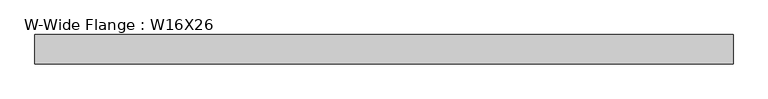
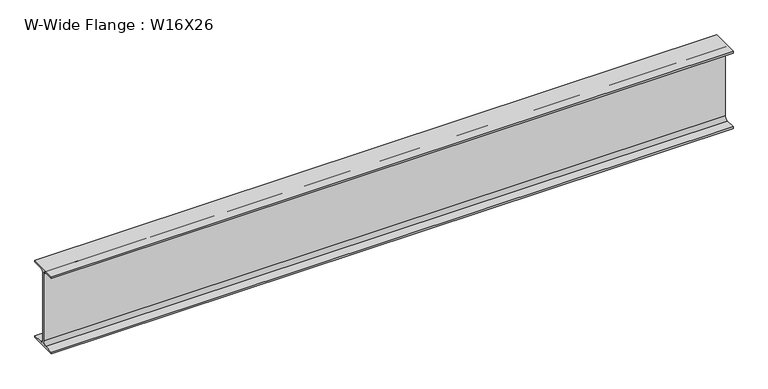
"""IFC4 building model written with IfcOpenShell, lengths in millimetres: beam geometry, W-Wide Flange : W16X26."""

from ifc_helpers import new_model, si_unit, point, frame, frame_2d, origin, place, context, project, spatial, polyline, circle_curve, trimmed, segment, composite_curve, outline, extrude, source, transform, mapped, element, save


def w_wide_flange_w16x26_c197a4b5(model_context):
    return source(origin(), model_context, "Body", "SweptSolid", [
        extrude(outline(composite_curve([segment(polyline([(69.85, -190.627), (69.85, -199.39), (-69.85, -199.39), (-69.85, -190.627), (-21.3995, -190.627)]), True, "CONTINUOUS"), segment(trimmed(circle_curve(frame_2d((-21.3995, -172.4025)), 18.2245), [point((-21.3995, -190.627))], [point((-3.175, -172.4025))], True, "CARTESIAN"), True, "CONTINUOUS"), segment(polyline([(-3.175, -172.4025), (-3.175, 172.4025)]), True, "CONTINUOUS"), segment(trimmed(circle_curve(frame_2d((-21.3995, 172.4025)), 18.2245), [point((-3.175, 172.4025))], [point((-21.3995, 190.627))], True, "CARTESIAN"), True, "CONTINUOUS"), segment(polyline([(-21.3995, 190.627), (-69.85, 190.627), (-69.85, 199.39), (69.85, 199.39), (69.85, 190.627), (21.3995, 190.627)]), True, "CONTINUOUS"), segment(trimmed(circle_curve(frame_2d((21.3995, 172.4025)), 18.2245), [point((21.3995, 190.627))], [point((3.175, 172.4025))], True, "CARTESIAN"), True, "CONTINUOUS"), segment(polyline([(3.175, 172.4025), (3.175, -172.4025)]), True, "CONTINUOUS"), segment(trimmed(circle_curve(frame_2d((21.3995, -172.4025)), 18.2245), [point((3.175, -172.4025))], [point((21.3995, -190.627))], True, "CARTESIAN"), True, "CONTINUOUS"), segment(polyline([(21.3995, -190.627), (69.85, -190.627)]), True, "CONTINUOUS")], self_intersect=False)), frame((-1587.5, 0.0, 0.0), z_axis=(1.0, 0.0, 0.0), x_axis=(0.0, 1.0, 0.0)), (0.0, 0.0, 1.0), 3327.4),
    ])


if __name__ == "__main__":
    model = new_model("IFC4")
    model_context = context("Model", 3, world=origin())
    ifc_project = project(units=[si_unit("LENGTHUNIT", "METRE", prefix="MILLI")], contexts=[model_context])
    site = spatial("IfcSite", under=ifc_project)
    building = spatial("IfcBuilding", under=site)
    placement = place(None, origin())
    w_wide_flange_w16x26_shape = w_wide_flange_w16x26_c197a4b5(model_context)
    element("IfcBeam", 1, ObjectType="W-Wide Flange : W16X26", at=placement, inside=building, context=model_context, shape_type="MappedRepresentation", body=[
        mapped(w_wide_flange_w16x26_shape, transform((0.0, 0.0, 0.0), x_axis=(1.0, 0.0, 0.0), y_axis=(0.0, 1.0, 0.0), z_axis=(0.0, 0.0, 1.0))),
    ])
    save(model, "model.ifc")

# Revit data of these elements
# Type "W-Wide Flange : W16X26"
#   Assembly Code = "B10"
#   W = 26
#   Length [instance default] = 5' - 0"
#   bf = 0' - 5 1/2"
#   d = 1' - 3.7"
#   k = 0' - 1 1/16"
#   k2 = 0' - 0.7175"
#   tf = 0' - 0.345"
#   tw = 0' - 0 1/4"
#   A = 0.0533333 SF
#   Structural Material [instance default] = Steel ASTM A992
# Element 1 (IfcBeam, "W-Wide Flange : W16X26")
#   Structural Material = Steel ASTM A36
#   Materials on its faces: "Steel ASTM A36"
# Materials
#   "Steel ASTM A992": class "Metal", colour RGB 199 199 199, transparency 0, Description = "Structural steel 50ksi", Cost = 0
#   "Steel ASTM A36": class "Metal", colour RGB 199 199 199, transparency 0, Description = "Structural steel, ASTM A36 Grade B, mill finish", Cost = 0
